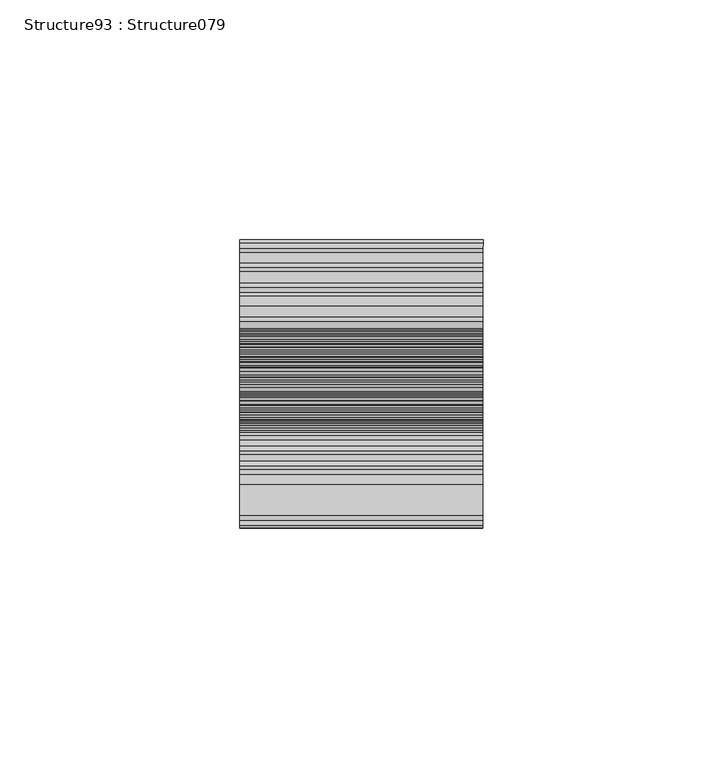
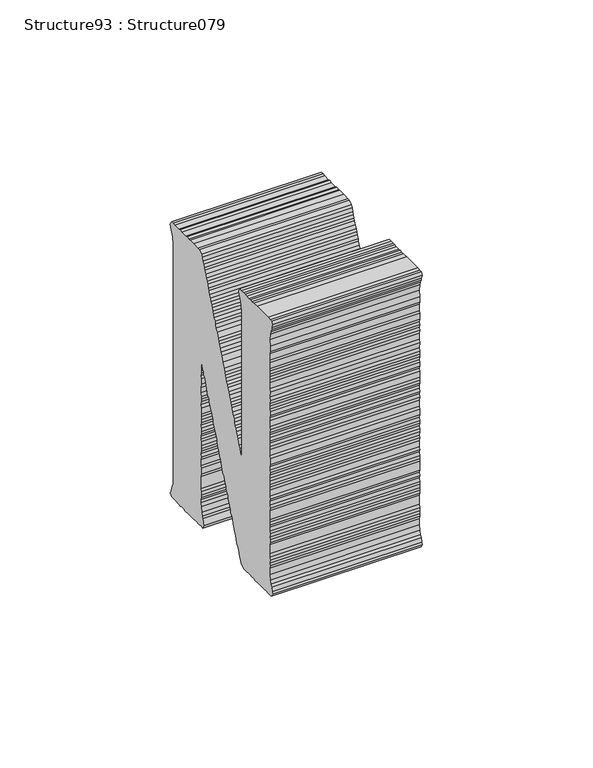
"""IFC4 building model written with IfcOpenShell, lengths in millimetres: proxy geometry, Structure93 : Structure079."""

from ifc_helpers import new_model, si_unit, frame, origin, place, context, project, spatial, polyline, outline, extrude, source, transform, mapped, element, save


def structure93_structure079_0899c1b0(model_context):
    return source(origin(), model_context, "Body", "SweptSolid", [
        extrude(outline(polyline([(1.8366799, 0.0), (3.1719919, 0.2053232), (3.9678799, 0.2224656), (6.1339986, 0.7044792), (7.2017339, -0.1002348), (6.9235449, -1.1141612), (6.9103347, -2.1601811), (6.6008944, -4.347663), (6.6194392, -5.1387182), (6.4560722, -6.2935847), (6.200152, -7.1805736), (6.164673, -8.353531), (5.8919629, -10.2813617), (5.504575, -11.1450817), (5.322519, -12.4320636), (5.4731793, -13.241808), (5.3278037, -14.2694911), (4.776401, -16.2926574), (4.4850018, -18.3526038), (3.4817959, -18.9944509), (2.4123488, -18.1891354), (1.5488816, -17.802502), (0.6787273, -17.4199537), (-0.4031239, -16.7429712), (-2.5708599, -16.3015648), (-3.6179366, -16.2882051), (-4.4817562, -15.9015219), (-5.5316583, -15.8827315), (-7.7145603, -15.573939), (-8.600592, -15.318873), (-9.646971, -15.300581), (-13.7622836, -14.7184305), (-14.8072465, -14.7053698), (-15.8412712, -14.5590971), (-16.8492085, -14.2817554), (-18.0093595, -14.1176409), (-19.0176422, -13.8452813), (-20.0827102, -13.9591049), (-20.8239266, -13.589765), (-22.015121, -13.6857468), (-23.1509461, -13.3903141), (-24.0757719, -13.394248), (-27.2905847, -12.9394818), (-28.3002834, -12.6618909), (-29.3265574, -12.5167146), (-30.11962, -12.5392877), (-31.3692171, -12.0980325), (-33.4665482, -12.0658325), (-34.4928222, -11.9206562), (-35.3742808, -11.6612061), (-36.5167928, -11.3698585), (-37.5628196, -11.3516163), (-38.4453282, -11.0970487), (-39.363467, -11.0968974), (-40.5405456, -11.0651477), (-42.5969688, -10.7742469), (-43.5925517, -10.3689245), (-44.6191778, -10.2236984), (-45.6838937, -10.3375718), (-46.5473609, -9.9509384), (-47.870671, -10.0282311), (-48.6260031, -9.7866228), (-49.6713184, -9.7735123), (-50.7947892, -9.3500989), (-51.9916205, -9.4452833), (-52.7233245, -9.0772891), (-53.9145189, -9.1732708), (-54.7818616, -8.7860892), (-56.1069332, -8.8631328), (-58.1672318, -8.5716838), (-59.0250621, -8.1858478), (-60.0943579, -8.2990733), (-61.0857131, -7.8943489), (-61.989736, -7.7664662), (-63.3091707, -7.8443072), (-64.3005258, -7.4395828), (-65.1151027, -7.5888408), (-66.1230399, -7.311499), (-67.2592105, -7.0210485), (-68.4193615, -6.856934), (-69.3565418, -6.9888485), (-70.5114082, -6.8254816), (-71.248749, -6.45669), (-72.4268915, -6.4197588), (-73.4774913, -6.4059006), (-74.6320055, -6.2425835), (-75.382053, -6.0017228), (-76.673615, -5.8190189), (-77.7189303, -5.8059084), (-78.7109901, -5.4010844), (-79.7608922, -5.382294), (-80.6391731, -5.1283244), (-81.7077643, -5.2416496), (-82.8298258, -4.8184355), (-83.6348904, -4.9690391), (-84.9045926, -4.6546682), (-85.695189, -4.6775901), (-88.0278455, -4.4773417), (-88.9646734, -4.609306), (-90.210194, -5.0867879), (-91.0208956, -5.236594), (-92.1011932, -5.4733198), (-93.1586381, -4.5399738), (-93.1207497, -3.3626856), (-92.7520508, -2.6310813), (-92.4419626, -0.4390194), (-92.5745818, 0.4982606), (-92.1872438, 1.3616281), (-91.8598122, 3.6762932), (-91.9924812, 4.6132209), (-91.587102, 5.604124), (-91.7377623, 6.4138683), (-91.4463133, 8.4741669), (-90.858928, 10.7516998), (-90.7315437, 11.6521997), (-89.7588844, 12.9570716), (-88.9361808, 13.2349082), (-87.6075862, 13.3114534), (-86.6587493, 13.5664164), (-85.7042825, 13.8256138), (-84.8931789, 13.9757224), (-83.775553, 14.4763272), (-82.5614281, 14.6937625), (-81.6062565, 14.9528603), (-80.6633896, 15.0843297), (-79.4362126, 15.434678), (-78.6501893, 15.4532158), (-77.5449109, 15.8208078), (-76.462154, 16.0622168), (-75.3808561, 16.3034729), (-74.534172, 16.7076455), (-73.5973441, 16.8396099), (-72.5104094, 17.0800685), (-71.6883537, 17.3533251), (-70.4908177, 17.4484098), (-69.4996705, 17.9669062), (-68.5635403, 18.0939382), (-67.3684206, 18.1897241), (-66.2493787, 18.6850974), (-64.4672759, 19.2214339), (-63.5102931, 19.4806348), (-62.4663801, 19.4626916), (-61.3649772, 19.8308319), (-60.1522683, 20.0534985), (-59.1790557, 20.4401319), (-57.1595208, 20.8131529), (-55.3756564, 21.3492402), (-54.1632432, 21.567277), (-53.2264153, 21.6992413), (-52.2712438, 21.9583392), (-51.0789855, 22.0491394), (-50.3414505, 22.603871), (-49.2971852, 22.585878), (-48.3063834, 23.0993922), (-47.1095521, 23.1945765), (-46.0042238, 23.5625208), (-45.0532801, 23.8222167), (-44.0981086, 24.0813146), (-43.3078576, 24.0992542), (-41.9482196, 24.4358957), (-40.9757116, 24.8226288), (-40.0205401, 25.0817265), (-38.9505328, 25.1898204), (-37.8872262, 25.3038932), (-37.0641205, 25.5820323), (-35.9782358, 25.8176084), (-34.8771851, 26.1857985), (-34.0315648, 26.5951527), (-32.0246798, 26.8355632), (-31.0754975, 27.0955082), (-29.7162049, 27.4271676), (-28.755699, 27.6858701), (-29.9749504, 28.3822892), (-32.0662924, 28.4136419), (-34.1269434, 28.7051408), (-34.8625227, 29.0736832), (-36.0187983, 29.2372495), (-37.0630636, 29.2552425), (-38.22709, 29.4199052), (-39.2741669, 29.4332649), (-40.0058708, 29.8012592), (-41.0748143, 29.6879838), (-42.0665217, 30.092758), (-43.098785, 30.2387816), (-44.289627, 30.1427499), (-45.171438, 30.4022499), (-46.4397241, 30.7113895), (-47.2320888, 30.6937487), (-48.2731764, 30.7062612), (-49.4008748, 31.1302726), (-50.4469016, 31.1485148), (-51.4555365, 31.4209243), (-53.5158352, 31.7123733), (-54.5844263, 31.5990481), (-56.5985323, 32.1484504), (-57.376429, 32.2584913), (-58.4418493, 32.1447176), (-59.7094377, 32.4587895), (-60.5003864, 32.4359174), (-61.5231373, 32.5805953), (-62.778019, 33.0225981), (-63.583436, 32.8720444), (-65.6440868, 33.1635432), (-66.9116752, 33.4776151), (-68.9719739, 33.7690641), (-69.8488455, 34.0228343), (-70.9195505, 33.9098082), (-71.8010091, 34.1692583), (-72.9555232, 34.3325754), (-74.1015584, 34.6244214), (-75.1479374, 34.6427134), (-75.9022058, 34.8791402), (-78.2475621, 34.9464257), (-79.2452588, 35.3520472), (-80.2711804, 35.4971736), (-82.2586151, 35.3840993), (-83.4696121, 35.1608312), (-84.40997, 35.0343972), (-85.6367948, 34.683999), (-86.7195018, 34.4429424), (-87.7897033, 35.2480052), (-87.5340788, 36.1303643), (-87.3520727, 37.416994), (-87.3342395, 38.4677503), (-86.9711776, 39.200152), (-86.7891714, 40.4867817), (-86.8981624, 41.5504475), (-86.5344526, 42.2874291), (-86.3883792, 43.3200447), (-86.3520443, 45.4110413), (-85.4425121, 51.8406668), (-85.0420721, 52.8372997), (-85.0228229, 53.8828246), (-83.9355358, 54.1232333), (-82.7042823, 53.5548448), (-81.9483022, 53.3178165), (-80.8660987, 52.6407841), (-79.8927349, 52.1088765), (-77.7426378, 51.540237), (-75.6456589, 51.5080868), (-73.7185328, 51.2354764), (-72.7233023, 50.8302038), (-70.5404003, 50.5214114), (-69.7476901, 50.5440342), (-67.5556282, 50.233946), (-66.5515663, 49.9571525), (-65.5062511, 49.944042), (-64.6191556, 49.6837945), (-63.5738403, 49.6706839), (-62.4323783, 49.3744538), (-60.3777166, 49.0838022), (-59.3066593, 49.1967786), (-57.288678, 48.646828), (-56.2200868, 48.7601532), (-55.0832117, 48.469603), (-54.1777794, 48.3415209), (-53.041602, 48.0460384), (-52.2365374, 48.196642), (-50.9442707, 48.0138384), (-50.0811559, 47.6272549), (-49.0358406, 47.6141443), (-46.8473017, 47.3045545), (-45.9252875, 47.3038551), (-44.7887646, 47.0133547), (-44.0390694, 46.7725438), (-43.0071585, 46.6265701), (-41.8318415, 46.5950695), (-40.9500307, 46.3355696), (-39.7733044, 46.3038697), (-38.6314901, 46.0075898), (-36.5771807, 45.716988), (-35.6400005, 45.8489025), (-33.5797018, 45.5574535), (-32.7102453, 45.1699729), (-31.4109159, 45.1209296), (-30.6245403, 45.1394176), (-29.6289575, 44.7340951), (-28.5822329, 44.7207852), (-27.5538452, 44.5753099), (-26.2823814, 44.2606898), (-25.4953081, 44.2841101), (-24.2256058, 43.9697392), (-22.1670688, 43.6785394), (-21.2298885, 43.8104539), (-20.3664213, 43.4238205), (-19.059341, 43.3736808), (-18.0094388, 43.3548904), (-17.1329195, 43.10117), (-13.9177544, 42.646354), (-13.030659, 42.3861065), (-11.8574559, 42.354905), (-11.1017713, 42.1132469), (-9.7968049, 42.0634062), (-9.0104293, 42.0818941), (-7.7421432, 41.7727545), (-6.8180151, 41.7717561), (-5.7917412, 41.6265798), (-4.9282739, 41.2399464), (-1.7131088, 40.7851304), (-0.5342688, 40.7531315), (0.3782332, 40.7537777), (1.5263822, 40.4616327), (2.3127577, 40.4801206), (3.4341147, 40.0570063), (5.6226535, 39.7474165), (7.4599813, 39.7519965), (8.7952933, 39.9573197), (9.6458529, 40.3609442), (10.9833286, 40.5663208), (11.7933325, 40.7111945), (12.8430266, 39.778945), (12.7156921, 38.8787974), (12.715498, 37.9552743), (12.4062518, 36.6913155), (12.2789173, 35.7911679), (11.982737, 34.6500582), (12.1333973, 33.840314), (11.8234534, 32.5714229), (11.6606399, 30.4983179), (11.273252, 29.634598), (11.3878799, 28.5701349), (10.9638616, 27.4474684), (10.8544685, 26.6741518), (10.9691462, 25.6100409), (10.6771936, 24.4683331), (10.5498093, 23.5678333), (9.4634279, 22.4091361), (8.5124343, 22.149088), (7.3955061, 21.6534155), (6.4713781, 21.654414), (5.2621923, 21.431249), (4.2833427, 21.045413), (3.3161693, 20.6582847), (2.1193378, 20.5631003), (1.0144118, 20.1954585), (-0.8952764, 19.6768108), (-1.8465726, 19.4171649), (-2.6424604, 19.4000225), (-3.9777726, 19.1946993), (-4.8065152, 18.9173575), (-5.9237956, 18.421735), (-6.8426322, 18.4169539), (-7.9493198, 18.0495612), (-8.9041889, 17.7900613), (-9.8713624, 17.4029329), (-11.0533802, 17.4404124), (-11.8951251, 17.03051), (-13.000101, 16.6625157), (-13.9147167, 16.6621687), (-15.0154151, 16.2939287), (-15.8243551, 16.1438733), (-16.9067666, 15.9074466), (-17.9021415, 15.3895482), (-19.94002, 14.8893938), (-20.9846376, 14.9074366), (-22.085738, 14.5388943), (-22.9183063, 14.262453), (-24.2373886, 14.1845622), (-26.0371803, 13.5206404), (-27.1258766, 13.2804309), (-28.0443677, 13.280632), (-29.2535535, 13.057467), (-30.0798369, 12.7848084), (-31.1812329, 12.4116362), (-31.990173, 12.2615808), (-33.2413305, 11.7848965), (-34.2873573, 11.8031387), (-35.3923332, 11.4351444), (-36.3235242, 11.3023827), (-37.4284502, 10.9347408), (-39.4663786, 10.434234), (-40.4025087, 10.307202), (-41.2622449, 9.7701163), (-42.2224055, 9.5163959), (-43.3033511, 9.27509), (-44.3722945, 9.1618147), (-45.1766614, 9.0161435), (-46.3861926, 8.7879963), (-47.5112736, 8.2931178), (-48.4484538, 8.1612034), (-49.2746874, 7.888897), (-50.3573944, 7.6478404), (-51.4623703, 7.2798462), (-50.4487962, 7.001707), (-49.5334827, 7.0069865), (-48.2419206, 6.8242826), (-47.3601098, 6.5647827), (-46.3514748, 6.2923733), (-45.4333359, 6.2922221), (-43.3726851, 6.0007232), (-42.1043989, 5.6915836), (-40.3037515, 5.4368648), (-38.9977212, 5.3818426), (-38.2106479, 5.4052629), (-37.1970738, 5.1271237), (-36.060551, 4.8366233), (-34.9954828, 4.9504469), (-32.8090579, 4.6411561), (-31.7954837, 4.363017), (-30.8766472, 4.3677981), (-29.740822, 4.0723654), (-28.8526765, 3.8170003), (-27.7897223, 3.9311229), (-26.6330943, 3.7675068), (-25.7477604, 3.5075085), (-24.8694795, 3.2535389), (-23.8372163, 3.1075153), (-22.9190774, 3.1073641), (-21.6324477, 2.925358), (-20.5857232, 2.9120481), (-19.577786, 2.6347064), (-18.6899928, 2.3793912), (-17.6249247, 2.4932147), (-16.5070909, 2.0705988), (-14.4485539, 1.7793989), (-13.5300626, 1.7791979), (-11.469764, 1.4877489), (-10.5876078, 1.2332311), (-6.2122917, 0.6143006), (-5.2997897, 0.6149468), (-4.1149604, 0.5821006), (-3.2204497, 0.4555635), (-2.3513456, 0.0681327), (-1.3247193, -0.0770934), (0.0, 0.0), (1.8366799, 0.0)])), frame((-56111.3579585, 291617.2747278, -368.3266136), z_axis=(-0.9999998917542984, 0.00046528635450596156, 0.0), x_axis=(-6.517039355318693e-05, -0.14006511446573924, -0.9901422925330072)), (0.0, 0.0, 1.0), 50.8),
    ])


if __name__ == "__main__":
    model = new_model("IFC4")
    model_context = context("Model", 3, world=origin())
    ifc_project = project(units=[si_unit("LENGTHUNIT", "METRE", prefix="MILLI")], contexts=[model_context])
    site = spatial("IfcSite", under=ifc_project)
    building = spatial("IfcBuilding", under=site)
    placement = place(None, origin())
    structure93_structure079_shape = structure93_structure079_0899c1b0(model_context)
    element("IfcBuildingElementProxy", 1, Name="Structure93 : Structure079", ObjectType="Structure93 : Structure079", at=placement, inside=building, context=model_context, shape_type="MappedRepresentation", body=[
        mapped(structure93_structure079_shape, transform((0.0, 0.0, 0.0), x_axis=(1.0, 0.0, 0.0), y_axis=(0.0, 1.0, 0.0), z_axis=(0.0, 0.0, 1.0))),
    ])
    save(model, "model.ifc")

# Revit data of these elements
# Type "Structure93 : Structure079"
#   NameOverride = "Structure079"
# Element 1 (IfcBuildingElementProxy, "Structure93 : Structure079")
#   Materials on its faces: "BRUSHED ALUMINUM LETTERING"
# Materials
#   "BRUSHED ALUMINUM LETTERING": class "Unassigned", colour RGB 169 181 186, transparency 0, Cost = 0
